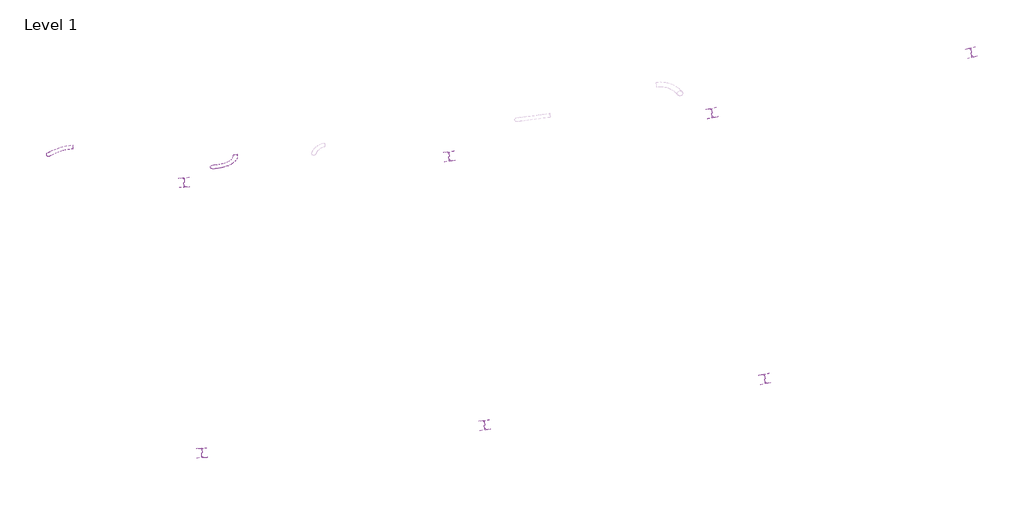
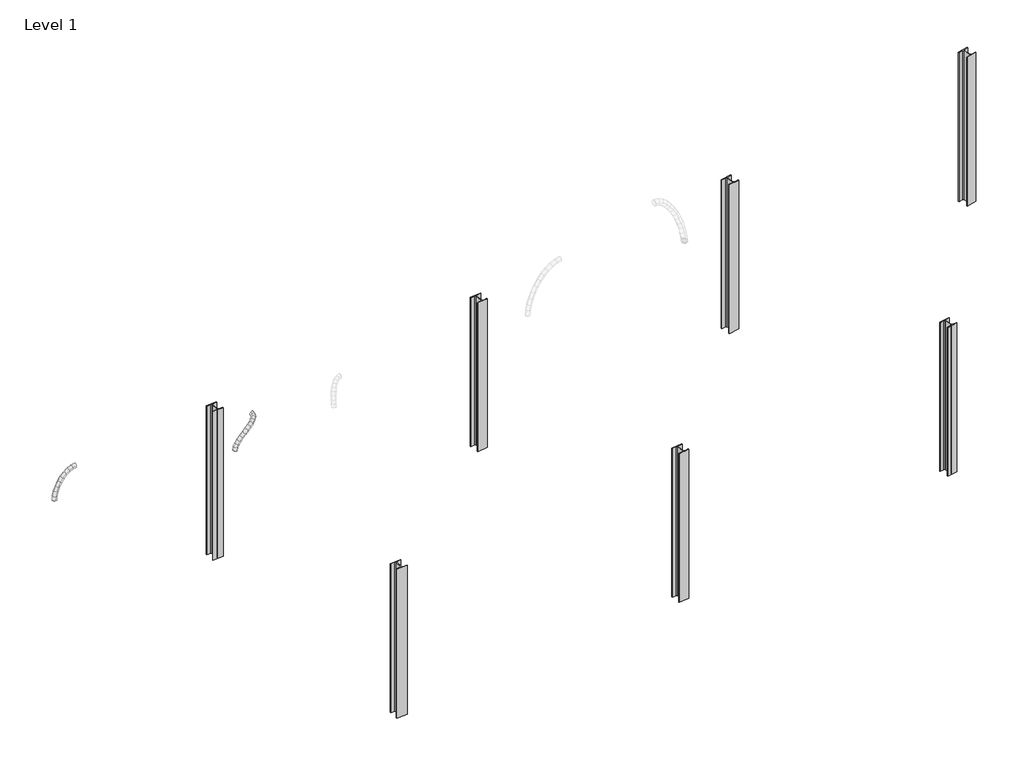
# One storey, part 1 of 3: 7 columns, 2 duct segments.
# Revit data of these elements (continued)
# Element 8 (IfcDuctSegment, "Flex - Round") (continued)
#   system = SA 32 (DUCT - SUPPLY AIR)
# Element 9 (IfcDuctSegment, "Flex - Round")
#   Mark = "641"
#   Phase Created = New Construction
#   section width or diameter = 0' - 6"
#   section height = 0' - 6"
#   system = SA 32 (DUCT - SUPPLY AIR)
# Materials
#   "Metal - Steel - ASTM A992": class "Metal", colour RGB 199 199 199, transparency 0
